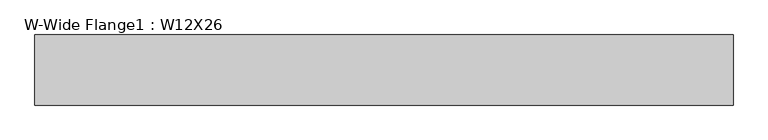
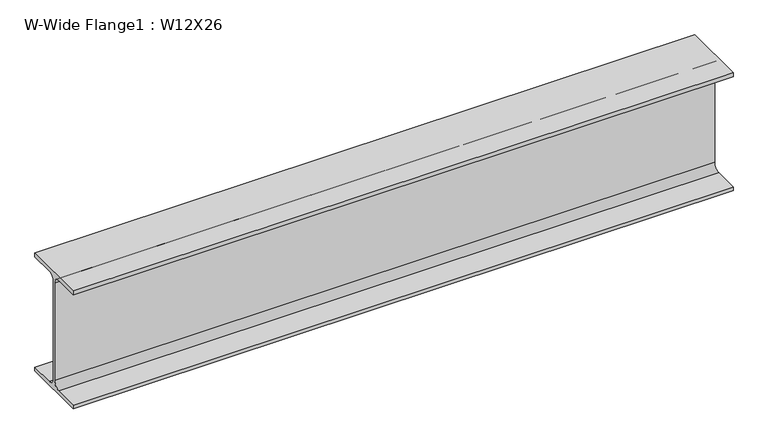
"""IFC4 building model written with IfcOpenShell, lengths in millimetres: beam geometry, W-Wide Flange1 : W12X26."""

import ifcopenshell
import ifcopenshell.guid

model = None  # the IFC model being written
_history = None  # IfcOwnerHistory: only IFC2X3 demands one
_inside = {}  # id of a spatial element -> (the spatial element, [elements in it])
_under = {}  # id of a project, library or spatial element -> (it, [spatial elements below it])
_declared = {}  # id of a project -> (the project, [libraries it declares])
_typed = {}  # id of a type object -> (the type object, [elements of that type])
_made_of = {}  # id of a material, layer set ... -> (it, [elements and type objects made of it])


def new_model(schema):
    """Start an empty IFC model of exactly this schema.

    Asked for "IFC4X3", IfcOpenShell would pick the latest addendum, in which some entities
    have other attributes; the version numbers below select the first issue.
    IFC2X3 requires an IfcOwnerHistory on every rooted entity: one is made here for all.
    """
    global model, _history
    if schema == "IFC4X3":
        model = ifcopenshell.file(schema_version=(4, 3, 0, 0))
    else:
        model = ifcopenshell.file(schema=schema)
    _inside.clear()
    _under.clear()
    _declared.clear()
    _typed.clear()
    _made_of.clear()
    _history = None
    if model.schema == "IFC2X3":
        org = make("IfcOrganization", Name="unknown")
        user = make(
            "IfcPersonAndOrganization",
            ThePerson=make("IfcPerson", FamilyName="unknown"),
            TheOrganization=org,
        )
        app = make(
            "IfcApplication",
            ApplicationDeveloper=org,
            Version="unknown",
            ApplicationFullName="unknown",
            ApplicationIdentifier="unknown",
        )
        _history = make(
            "IfcOwnerHistory",
            OwningUser=user,
            OwningApplication=app,
            ChangeAction="ADDED",
            CreationDate=0,
        )
    return model


def make(cls, **values):
    """One entity of the class cls with the attributes given. An attribute that is None is left unset."""
    return model.create_entity(
        cls, **{name: value for name, value in values.items() if value is not None}
    )


def rooted(cls, **values):
    """An entity with a GlobalId (a new one), such as an element, a storey or a relation."""
    return make(cls, GlobalId=ifcopenshell.guid.new(), OwnerHistory=_history, **values)


def si_unit(unit_type, name, prefix=None):
    """IfcSIUnit, for example si_unit("LENGTHUNIT", "METRE", prefix="MILLI")."""
    return make("IfcSIUnit", UnitType=unit_type, Prefix=prefix, Name=name)


def assignment(units):
    """IfcUnitAssignment: the units of a project."""
    return None if units is None else make("IfcUnitAssignment", Units=units)


def point(xyz):
    """IfcCartesianPoint."""
    return None if xyz is None else make("IfcCartesianPoint", Coordinates=xyz)


def direction(xyz):
    """IfcDirection."""
    return None if xyz is None else make("IfcDirection", DirectionRatios=xyz)


def frame(location, z_axis=None, x_axis=None):
    """IfcAxis2Placement3D, a coordinate frame: its origin and axes. An axis left out is left unset."""
    return make(
        "IfcAxis2Placement3D",
        Location=point(location),
        Axis=direction(z_axis),
        RefDirection=direction(x_axis),
    )


def frame_2d(location, x_axis=None):
    """IfcAxis2Placement2D, a coordinate frame in the plane: its origin and x axis."""
    return make(
        "IfcAxis2Placement2D", Location=point(location), RefDirection=direction(x_axis)
    )


def origin():
    """The frame at (0, 0, 0) with its axes left unset."""
    return frame((0.0, 0.0, 0.0))


def place(relative_to, where):
    """IfcLocalPlacement: puts the frame where relative to a parent placement (None: the world)."""
    return make(
        "IfcLocalPlacement", PlacementRelTo=relative_to, RelativePlacement=where
    )


def context(
    kind, dimensions, precision=None, world=None, true_north=None, identifier=None
):
    """IfcGeometricRepresentationContext, for example the 3D "Model" context."""
    return make(
        "IfcGeometricRepresentationContext",
        ContextIdentifier=identifier,
        ContextType=kind,
        CoordinateSpaceDimension=dimensions,
        Precision=precision,
        WorldCoordinateSystem=world,
        TrueNorth=true_north,
    )


def project(units=None, contexts=None):
    """IfcProject with its units and contexts."""
    return rooted(
        "IfcProject",
        Name="project",
        RepresentationContexts=contexts,
        UnitsInContext=assignment(units),
    )


def spatial(cls, under=None, at=None, **own):
    """A site, building, storey or space (cls), placed at a placement, below another one or the project."""
    s = rooted(cls, ObjectPlacement=at, **own)
    if under is not None:
        _under.setdefault(under.id(), (under, []))[1].append(s)
    return s


def polyline(points):
    """IfcPolyline through the points."""
    return make("IfcPolyline", Points=[point(p) for p in points])


def circle_curve(where, radius):
    """IfcCircle in the frame where."""
    return make("IfcCircle", Position=where, Radius=radius)


def trimmed(basis, trim1, trim2, sense, master):
    """IfcTrimmedCurve: the piece of a basis curve between two trims."""
    return make(
        "IfcTrimmedCurve",
        BasisCurve=basis,
        Trim1=trim1,
        Trim2=trim2,
        SenseAgreement=sense,
        MasterRepresentation=master,
    )


def segment(curve, same_sense, transition):
    """IfcCompositeCurveSegment."""
    return make(
        "IfcCompositeCurveSegment",
        Transition=transition,
        SameSense=same_sense,
        ParentCurve=curve,
    )


def composite_curve(segments, self_intersect=None):
    """IfcCompositeCurve: segments joined end to end."""
    return make("IfcCompositeCurve", Segments=segments, SelfIntersect=self_intersect)


def outline(outer, holes=None, kind="AREA"):
    """IfcArbitraryClosedProfileDef: a profile drawn as a closed curve; with holes, ...WithVoids."""
    if holes is None:
        return make("IfcArbitraryClosedProfileDef", ProfileType=kind, OuterCurve=outer)
    return make(
        "IfcArbitraryProfileDefWithVoids",
        ProfileType=kind,
        OuterCurve=outer,
        InnerCurves=holes,
    )


def extrude(swept, where, along, depth):
    """IfcExtrudedAreaSolid: the profile swept, set in the frame where, extruded along a direction by depth."""
    return make(
        "IfcExtrudedAreaSolid",
        SweptArea=swept,
        Position=where,
        ExtrudedDirection=direction(along),
        Depth=depth,
    )


def shape(context_of_items, identifier, shape_type, items):
    """IfcShapeRepresentation: the items that make up one representation, for example the "Body"."""
    return make(
        "IfcShapeRepresentation",
        ContextOfItems=context_of_items,
        RepresentationIdentifier=identifier,
        RepresentationType=shape_type,
        Items=items,
    )


def source(mapping_origin, context_of_items, identifier, shape_type, items):
    """IfcRepresentationMap: a shape defined once, which mapped items show again and again."""
    return make(
        "IfcRepresentationMap",
        MappingOrigin=mapping_origin,
        MappedRepresentation=shape(context_of_items, identifier, shape_type, items),
    )


def transform(
    local_origin,
    x_axis=None,
    y_axis=None,
    z_axis=None,
    scale=None,
    scale2=None,
    scale3=None,
    uniform=True,
):
    """IfcCartesianTransformationOperator3D, or its non-uniform kind. x_axis, y_axis, z_axis: its Axis1, 2, 3."""
    if uniform:
        return make(
            "IfcCartesianTransformationOperator3D",
            Axis1=direction(x_axis),
            Axis2=direction(y_axis),
            LocalOrigin=point(local_origin),
            Scale=scale,
            Axis3=direction(z_axis),
        )
    return make(
        "IfcCartesianTransformationOperator3DnonUniform",
        Axis1=direction(x_axis),
        Axis2=direction(y_axis),
        LocalOrigin=point(local_origin),
        Scale=scale,
        Axis3=direction(z_axis),
        Scale2=scale2,
        Scale3=scale3,
    )


def mapped(mapping_source, mapping_target):
    """IfcMappedItem: shows the shape of a source again, moved by a transform."""
    return make(
        "IfcMappedItem", MappingSource=mapping_source, MappingTarget=mapping_target
    )


def made_of(thing, what):
    """Note that an element or type object is made of a material, layer set ...; save() writes the relation."""
    if what is not None:
        _made_of.setdefault(what.id(), (what, []))[1].append(thing)
    return thing


def element(
    cls,
    number,
    at=None,
    inside=None,
    cuts=None,
    type_object=None,
    material=None,
    context=None,
    identifier="Body",
    shape_type=None,
    held_by="IfcProductDefinitionShape",
    body=None,
    shapes=None,
    **own,
):
    """One element of the class cls, such as IfcWall. Its Tag is "e" and its number.

    at: its placement. inside: the storey or other place that contains it. cuts: it is an
    opening in that element (IfcRelVoidsElement). A single representation is given by context,
    identifier, shape_type and body (its items); several are given by shapes. held_by: the class
    of the entity that holds the representations. save() writes the other relations.
    """
    e = rooted(cls, Tag="e%d" % number, ObjectPlacement=at, **own)
    if body is not None:
        shapes = [shape(context, identifier, shape_type, body)]
    if shapes is not None:
        e.Representation = make(held_by, Representations=shapes)
    if inside is not None:
        _inside.setdefault(inside.id(), (inside, []))[1].append(e)
    if cuts is not None:
        rooted(
            "IfcRelVoidsElement", RelatingBuildingElement=cuts, RelatedOpeningElement=e
        )
    if type_object is not None:
        _typed.setdefault(type_object.id(), (type_object, []))[1].append(e)
    return made_of(e, material)


def aggregate(whole, parts):
    """IfcRelAggregates: a whole, such as a stair, and the parts it consists of."""
    return rooted("IfcRelAggregates", RelatingObject=whole, RelatedObjects=parts)


def save(model, path):
    """Write the relations noted so far, then the file.

    IfcRelAggregates (storeys below a building ...), IfcRelContainedInSpatialStructure (elements
    in a storey), IfcRelDefinesByType, IfcRelAssociatesMaterial and IfcRelDeclares: one each for
    every whole, place, type object, material and project.
    """
    for whole, parts in _under.values():
        aggregate(whole, parts)
    for where, things in _inside.values():
        rooted(
            "IfcRelContainedInSpatialStructure",
            RelatedElements=things,
            RelatingStructure=where,
        )
    for kind, things in _typed.values():
        rooted("IfcRelDefinesByType", RelatedObjects=things, RelatingType=kind)
    for what, things in _made_of.values():
        rooted("IfcRelAssociatesMaterial", RelatedObjects=things, RelatingMaterial=what)
    for by, libraries in _declared.values():
        rooted("IfcRelDeclares", RelatingContext=by, RelatedDefinitions=libraries)
    model.write(path)


def w_wide_flange1_w12x26_20602fd0(model_context):
    return source(origin(), model_context, "Body", "SweptSolid", [
        extrude(outline(composite_curve([segment(polyline([(82.423, -145.288), (82.423, -154.94), (-82.423, -154.94), (-82.423, -145.288), (-20.2565, -145.288)]), True, "CONTINUOUS"), segment(trimmed(circle_curve(frame_2d((-20.2565, -127.9525)), 17.3355), [point((-20.2565, -145.288))], [point((-2.921, -127.9525))], True, "CARTESIAN"), True, "CONTINUOUS"), segment(polyline([(-2.921, -127.9525), (-2.921, 127.9525)]), True, "CONTINUOUS"), segment(trimmed(circle_curve(frame_2d((-20.2565, 127.9525)), 17.3355), [point((-2.921, 127.9525))], [point((-20.2565, 145.288))], True, "CARTESIAN"), True, "CONTINUOUS"), segment(polyline([(-20.2565, 145.288), (-82.423, 145.288), (-82.423, 154.94), (82.423, 154.94), (82.423, 145.288), (20.2565, 145.288)]), True, "CONTINUOUS"), segment(trimmed(circle_curve(frame_2d((20.2565, 127.9525)), 17.3355), [point((20.2565, 145.288))], [point((2.921, 127.9525))], True, "CARTESIAN"), True, "CONTINUOUS"), segment(polyline([(2.921, 127.9525), (2.921, -127.9525)]), True, "CONTINUOUS"), segment(trimmed(circle_curve(frame_2d((20.2565, -127.9525)), 17.3355), [point((2.921, -127.9525))], [point((20.2565, -145.288))], True, "CARTESIAN"), True, "CONTINUOUS"), segment(polyline([(20.2565, -145.288), (82.423, -145.288)]), True, "CONTINUOUS")], self_intersect=False)), frame((-762.689828, 0.0, 0.0), z_axis=(1.0, 0.0, 0.0), x_axis=(0.0, 1.0, 0.0)), (0.0, 0.0, 1.0), 1641.2402705),
    ])


if __name__ == "__main__":
    model = new_model("IFC4")
    model_context = context("Model", 3, world=origin())
    ifc_project = project(units=[si_unit("LENGTHUNIT", "METRE", prefix="MILLI")], contexts=[model_context])
    site = spatial("IfcSite", under=ifc_project)
    building = spatial("IfcBuilding", under=site)
    placement = place(None, origin())
    w_wide_flange1_w12x26_shape = w_wide_flange1_w12x26_20602fd0(model_context)
    element("IfcBeam", 1, ObjectType="W-Wide Flange1 : W12X26", at=placement, inside=building, context=model_context, shape_type="MappedRepresentation", body=[
        mapped(w_wide_flange1_w12x26_shape, transform((0.0, 0.0, 0.0), x_axis=(1.0, 0.0, 0.0), y_axis=(0.0, 1.0, 0.0), z_axis=(0.0, 0.0, 1.0))),
    ])
    save(model, "model.ifc")

# Revit data of these elements
# Type "W-Wide Flange1 : W12X26"
#   Assembly Code = "B10"
#   W = 26
#   Start Extension Calculation [instance default] = 10' - 0"
#   Start Extension [instance default] = -0' - 0 1/2"
#   End Extension Calculation [instance default] = 10' - 0"
#   End Extension [instance default] = -0' - 0 1/2"
#   Length [instance default] = 5' - 0"
#   bf = 0' - 6.49"
#   d = 1' - 0.2"
#   k = 0' - 1 1/16"
#   k2 = 0' - 0.6825"
#   tf = 0' - 0.38"
#   tw = 0' - 0.23"
#   A = 0.053125 SF
#   Structural Material [instance default] = Metal - Steel - ASTM A992
# Element 1 (IfcBeam, "W-Wide Flange1 : W12X26")
#   Materials on its faces: "Metal - Steel - ASTM A992"
# Materials
#   "Metal - Steel - ASTM A992": class "Metal", colour RGB 199 199 199, transparency 0
